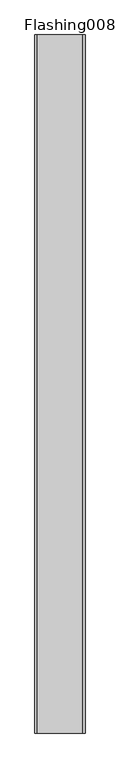
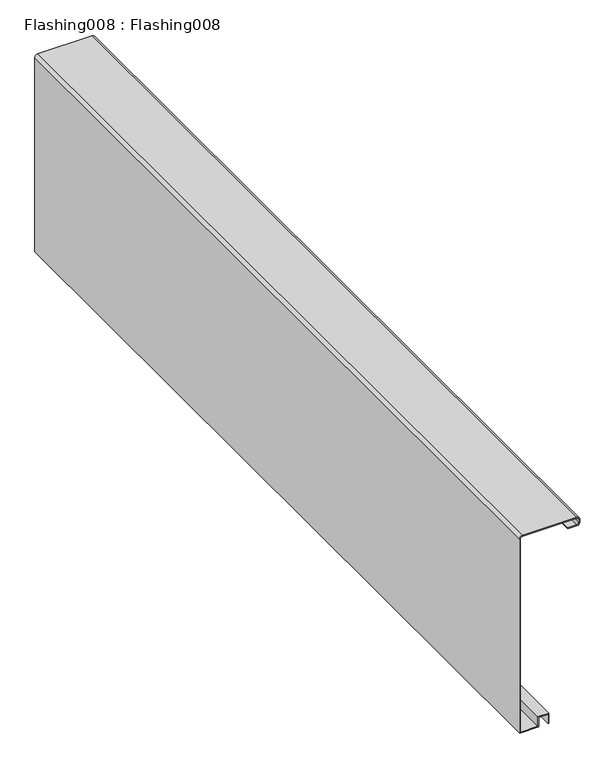
"""IFC4 building model written with IfcOpenShell, lengths in millimetres: proxy geometry, Flashing008 : Flashing008."""

from ifc_helpers import new_model, si_unit, point, frame, frame_2d, origin, place, context, project, spatial, polyline, circle_curve, trimmed, segment, composite_curve, outline, extrude, source, transform, mapped, element, save


def flashing008_flashing008_3e815ed5(model_context):
    return source(origin(), model_context, "Body", "SweptSolid", [
        extrude(outline(composite_curve([segment(trimmed(circle_curve(frame_2d((43518.4785937, -6493.7749805)), 5.08), [point((43518.4785937, -6498.8549805))], [point((43523.5585937, -6493.7749805))], True, "CARTESIAN"), True, "CONTINUOUS"), segment(polyline([(43523.5585937, -6493.7749805), (43523.5585937, -6364.4349805)]), True, "CONTINUOUS"), segment(trimmed(circle_curve(frame_2d((43518.4785937, -6364.4349805)), 5.08), [point((43523.5585937, -6364.4349805))], [point((43518.4785937, -6359.3549805))], True, "CARTESIAN"), True, "CONTINUOUS"), segment(polyline([(43518.4785937, -6359.3549805), (43512.0721875, -6359.3549805)]), True, "CONTINUOUS"), segment(trimmed(circle_curve(frame_2d((43512.0721875, -6364.4349805)), 5.08), [point((43512.0721875, -6359.3549805))], [point((43506.9921875, -6364.4349805))], True, "CARTESIAN"), True, "CONTINUOUS"), segment(polyline([(43506.9921875, -6364.4349805), (43506.9921875, -6385.7314453), (43504.9921875, -6385.7314453), (43504.9921875, -6364.4349805)]), True, "CONTINUOUS"), segment(trimmed(circle_curve(frame_2d((43512.0721875, -6364.4349805)), 7.08), [point((43504.9921875, -6364.4349805))], [point((43512.0721875, -6357.3549805))], False, "CARTESIAN"), True, "CONTINUOUS"), segment(polyline([(43512.0721875, -6357.3549805), (43518.4785937, -6357.3549805)]), True, "CONTINUOUS"), segment(trimmed(circle_curve(frame_2d((43518.4785937, -6364.4349805)), 7.08), [point((43518.4785937, -6357.3549805))], [point((43525.5585937, -6364.4349805))], False, "CARTESIAN"), True, "CONTINUOUS"), segment(polyline([(43525.5585937, -6364.4349805), (43525.5585937, -6493.7749805)]), True, "CONTINUOUS"), segment(trimmed(circle_curve(frame_2d((43518.4785937, -6493.7749805)), 7.08), [point((43525.5585937, -6493.7749805))], [point((43518.4785937, -6500.8549805))], False, "CARTESIAN"), True, "CONTINUOUS"), segment(polyline([(43518.4785937, -6500.8549805), (43030.1617235, -6500.8549805), (43030.1617235, -6455.5298267), (43054.2082994, -6455.5298267), (43054.2082994, -6433.1296096), (43030.1617235, -6433.1296096), (43030.1617235, -6431.1296096), (43056.2082994, -6431.1296096), (43056.2082994, -6457.5298267), (43032.1617235, -6457.5298267), (43032.1617235, -6498.8549805), (43518.4785937, -6498.8549805)]), True, "CONTINUOUS")], self_intersect=False)), frame((0.0, 7982.1531721, 0.0), z_axis=(0.0, 1.0, 0.0), x_axis=(0.0, 0.0, 1.0)), (0.0, 0.0, 1.0), 2000.0),
    ])


if __name__ == "__main__":
    model = new_model("IFC4")
    model_context = context("Model", 3, world=origin())
    ifc_project = project(units=[si_unit("LENGTHUNIT", "METRE", prefix="MILLI")], contexts=[model_context])
    site = spatial("IfcSite", under=ifc_project)
    building = spatial("IfcBuilding", under=site)
    placement = place(None, origin())
    flashing008_flashing008_shape = flashing008_flashing008_3e815ed5(model_context)
    element("IfcBuildingElementProxy", 1, Name="Flashing008 : Flashing008", ObjectType="Flashing008 : Flashing008", at=placement, inside=building, context=model_context, shape_type="MappedRepresentation", body=[
        mapped(flashing008_flashing008_shape, transform((0.0, 0.0, 0.0), x_axis=(1.0, 0.0, 0.0), y_axis=(0.0, 1.0, 0.0), z_axis=(0.0, 0.0, 1.0))),
    ])
    save(model, "model.ifc")

# Revit data of these elements
# Type "Flashing008 : Flashing008"
#   NameOverride = "Flashing008"
# Element 1 (IfcBuildingElementProxy, "Flashing008 : Flashing008")
#   Materials on its faces: "BRAKE METAL EAVE TRIM TO MATCH STANDING SEAM COLOR"
# Materials
#   "BRAKE METAL EAVE TRIM TO MATCH STANDING SEAM COLOR": class "Unassigned", colour RGB 128 128 128, transparency 0, Cost = 0
